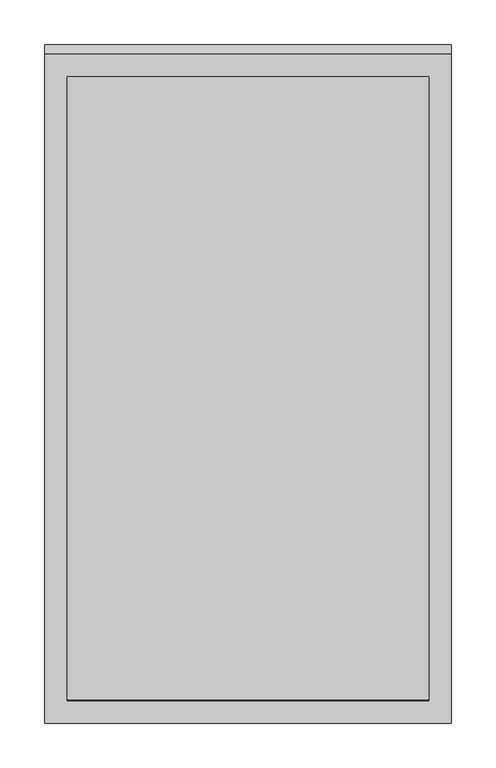
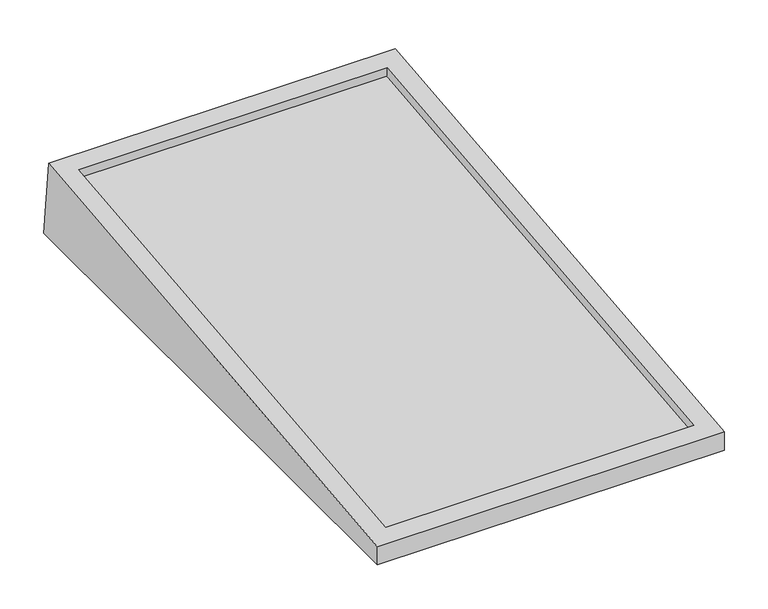
"""IFC4 building model written with IfcOpenShell, lengths in millimetres: proxy geometry, Bradley-Washroom_Accessories-Mirrors-740_Custom : Bradley-Washroom_Accessories-Mirrors-740_Custom."""

from ifc_helpers import new_model, si_unit, origin, place, context, project, spatial, faceted_brep, source, transform, mapped, element, save


def specialty_equipment_9c1522b1(model_context):
    return source(origin(), model_context, "Body", "Brep", [
        faceted_brep([(228.6, -381.0, 0.0), (228.6, 381.0, 0.0), (228.6, 370.0337574, 104.3368287), (228.6, -381.0, 25.4), (-228.6, -381.0, 0.0), (-228.6, -381.0, 25.4), (-228.6, 370.0337574, 104.3368287), (-228.6, 381.0, 0.0), (-203.2, -355.7391439, 28.055023), (-203.2, 344.7729013, 101.6818058), (203.2, 344.7729013, 101.6818058), (203.2, -355.7391439, 28.055023), (-203.2, -354.4116324, 15.4245949), (203.2, -354.4116324, 15.4245949), (203.2, 346.1004127, 89.0513777), (-203.2, 346.1004127, 89.0513777)], [[[0, 1, 2, 3]], [[4, 5, 6, 7]], [[1, 0, 4, 7]], [[2, 1, 7, 6]], [[3, 2, 6, 5], [8, 9, 10, 11]], [[0, 3, 5, 4]], [[12, 13, 14, 15]], [[12, 15, 9, 8]], [[15, 14, 10, 9]], [[14, 13, 11, 10]], [[13, 12, 8, 11]]]),
    ])


if __name__ == "__main__":
    model = new_model("IFC4")
    model_context = context("Model", 3, world=origin())
    ifc_project = project(units=[si_unit("LENGTHUNIT", "METRE", prefix="MILLI")], contexts=[model_context])
    site = spatial("IfcSite", under=ifc_project)
    building = spatial("IfcBuilding", under=site)
    placement = place(None, origin())
    specialty_equipment_shape = specialty_equipment_9c1522b1(model_context)
    element("IfcBuildingElementProxy", 1, Name="Bradley-Washroom_Accessories-Mirrors-740_Custom : Bradley-Washroom_Accessories-Mirrors-740_Custom", ObjectType="Bradley-Washroom_Accessories-Mirrors-740_Custom : Bradley-Washroom_Accessories-Mirrors-740_Custom", at=placement, inside=building, context=model_context, shape_type="MappedRepresentation", body=[
        mapped(specialty_equipment_shape, transform((0.0, 0.0, 0.0), x_axis=(1.0, 0.0, 0.0), y_axis=(0.0, 1.0, 0.0), z_axis=(0.0, 0.0, 1.0))),
    ])
    save(model, "model.ifc")

# Revit data of these elements
# Type "Bradley-Washroom_Accessories-Mirrors-740_Custom : Bradley-Washroom_Accessories-Mirrors-740_Custom"
#   Warranty Information = "Complete unit, excepting mirrors warranted for one year.\r\n Stainless steel mirror frames for fifteen years.\r\n Plate glass mirrors for fifteen years.\r\n This warranty does not cover installation or any other labor charges and does not apply to any units,\r\n which have been damaged by accident, abuse, improper installation, improper maintenance, or altered in any way."
#   Version = "1.0"
#   URL = "http://www.bradleycorp.com/"
#   Type Comments = "ERROR - If you are able to see this message you haven't loaded this  family correctly."
#   OmniClass Title = "Mirrors"
#   OmniClass Code = "23.40.95.17.17"
#   Modeling Code = ""
#   Model = "740-A"
#   MasterFormat Title = "Commercial Toilet Accessories"
#   MasterFormat Number = "10 28 13. 13"
#   Manufacturer = "Bradley Corporation"
#   Industry Standards = "ASTM C 1036"
#   Fire Rating = "n/a"
#   Dimensional Limits [instance default] = "Either Width or Hight must be over 25\""
#   Description = "ERROR - If you are able to see this message you haven't loaded this  family correctly."
#   Copyright = "This Model Data is Property of Bradley Corporation"
#   Buy American Act = "Yes"
#   Assembly Code = "C1030900"
#   ADA Compliant = "Yes"
#   Width [instance default] = 457.2 mm
#   Total Width [instance default] = 457.2 mm
#   Total Height [instance default] = 762 mm
#   Total Depth [instance default] = 105.051 mm
#   Height [instance default] = 762 mm
#   Depth [instance default] = 105.051 mm
#   Default Elevation = 1016 mm
#   Reflective Material = Glass - Bradley Corp - BradEX - Polished Float Mirror
#   Frame Material = Bradley Corp Stainless Steel - Satin
# Element 1 (IfcBuildingElementProxy, "Bradley-Washroom_Accessories-Mirrors-740_Custom : Bradley-Washroom_Accessories-Mirrors-740_Custom")
#   Materials on its faces: "Bradley Corp Stainless Steel - Satin"
# Materials
#   "Glass - Bradley Corp - BradEX - Polished Float Mirror": class "Glass", colour RGB 220 232 220, transparency 0, Manufacturer = "Bradley Corporation", URL = "www.bradleycorp.com", Description = "Stainless Steel - Satin Finish", Cost = 0
#   "Bradley Corp Stainless Steel - Satin": class "Metal", colour RGB 189 187 185, transparency 0, Manufacturer = "Bradley Corporation", URL = "www.bradleycorp.com", Description = "Stainless Steel - Satin Finish", Cost = 0
